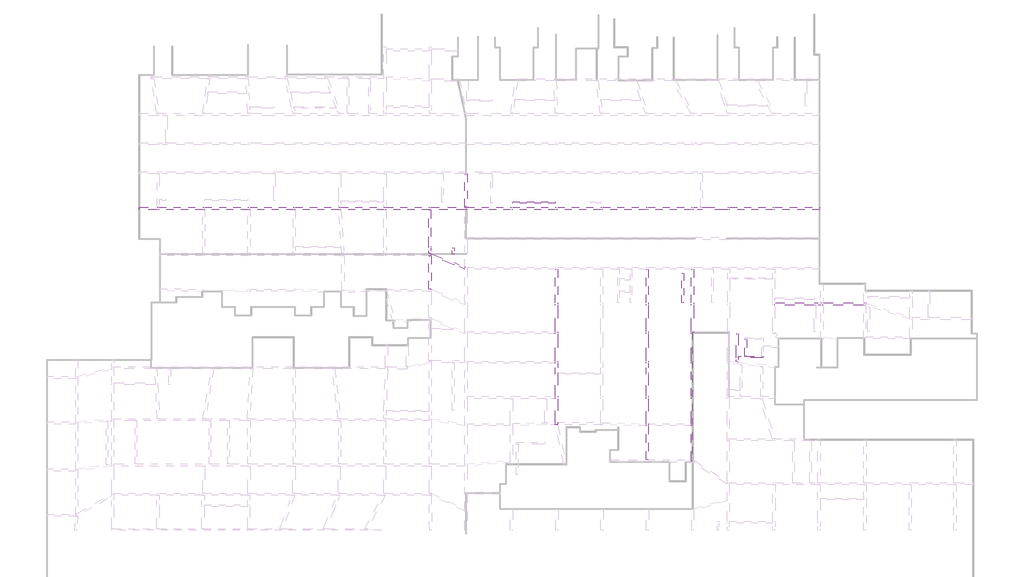
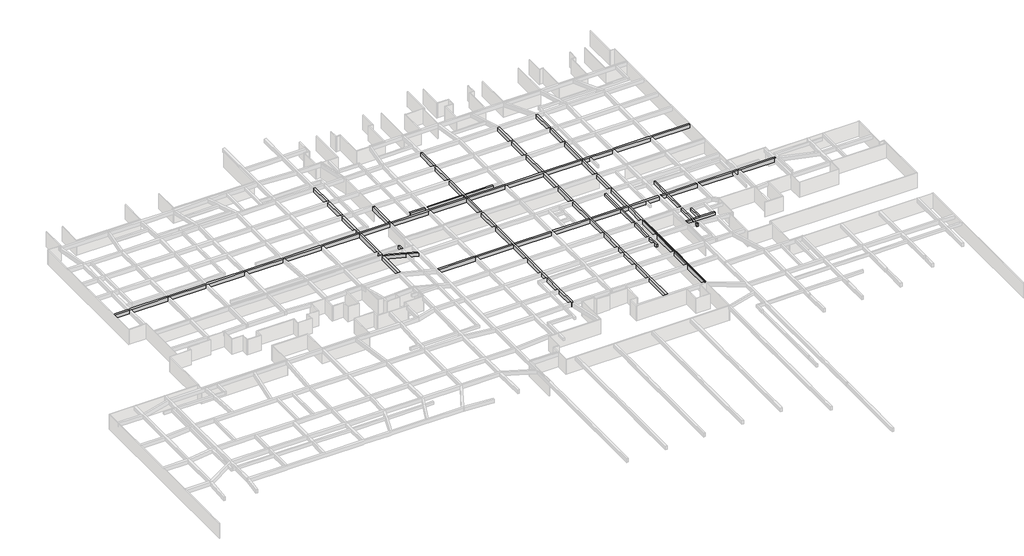
# One storey, part 14 of 16: 15 beams.
"""IFC4 building model written with IfcOpenShell, lengths in millimetres."""

from ifc_helpers import new_model, si_unit, frame, origin, place, context, project, spatial, polyline, outline, extrude, faceted_brep, element, save

model = new_model("IFC4")

# Units and contexts
model_context = context("Model", 3, world=origin())
ifc_project = project(units=[si_unit("LENGTHUNIT", "METRE", prefix="MILLI")], contexts=[model_context])

# Site, building, storey
site = spatial("IfcSite", under=ifc_project)
building = spatial("IfcBuilding", under=site)
storey = spatial("IfcBuildingStorey", under=building, Name="户型图", Elevation=0.0)

# Beams
placement = place(None, origin())
element("IfcBeam", 1, ObjectType="混凝土 - 矩形梁 : KL_beam", at=placement, inside=storey, context=model_context, shape_type="Brep", body=[
    faceted_brep([(204626.2466536, 173512.5884701, 3300.0), (204626.2466536, 173112.5884701, 3300.0), (204626.2466536, 173112.5884701, 2500.0), (204626.2466536, 173512.5884701, 2500.0), (83129.2466536, 173512.5884701, 3300.0), (83129.2466536, 173512.5884701, 2500.0), (83129.2466536, 173112.5884701, 2500.0), (83129.2466536, 173112.5884701, 3300.0), (196626.5590225, 173512.5884701, 3300.0), (196226.5590225, 173512.5884701, 3300.0), (188616.2109037, 173512.5884701, 3300.0), (188216.2109037, 173512.5884701, 3300.0), (183653.5662503, 173512.5884701, 3300.0), (183353.5662503, 173512.5884701, 3300.0), (182116.2109037, 173512.5884701, 3300.0), (181716.2109037, 173512.5884701, 3300.0), (174016.2109037, 173512.5884701, 3300.0), (173616.2109037, 173512.5884701, 3300.0), (165916.2109037, 173512.5884701, 3300.0), (165516.2109037, 173512.5884701, 3300.0), (157816.2109037, 173512.5884701, 3300.0), (157416.2109037, 173512.5884701, 3300.0), (149816.2109037, 173512.5884701, 3300.0), (149416.2109037, 173512.5884701, 3300.0), (141660.1899051, 173512.5884701, 3300.0), (141260.1899051, 173512.5884701, 3300.0), (135216.2109037, 173512.5884701, 3300.0), (134816.2109037, 173512.5884701, 3300.0), (127216.2109037, 173512.5884701, 3300.0), (126816.2109037, 173512.5884701, 3300.0), (119116.2109037, 173512.5884701, 3300.0), (118716.2109037, 173512.5884701, 3300.0), (111016.2109037, 173512.5884701, 3300.0), (110616.2109037, 173512.5884701, 3300.0), (102916.2109037, 173512.5884701, 3300.0), (102516.2109037, 173512.5884701, 3300.0), (94816.2109037, 173512.5884701, 3300.0), (94416.2109037, 173512.5884701, 3300.0), (86694.1615746, 173512.5884701, 3300.0), (86294.1615746, 173512.5884701, 3300.0), (86294.1615746, 173112.5884701, 3300.0), (86694.1615746, 173112.5884701, 3300.0), (94416.2109037, 173112.5884701, 3300.0), (94816.2109037, 173112.5884701, 3300.0), (102516.2109037, 173112.5884701, 3300.0), (102916.2109037, 173112.5884701, 3300.0), (110616.2109037, 173112.5884701, 3300.0), (111016.2109037, 173112.5884701, 3300.0), (118729.7078864, 173112.5884701, 3300.0), (119130.6846457, 173112.5884701, 3300.0), (126816.2109037, 173112.5884701, 3300.0), (127216.2109037, 173112.5884701, 3300.0), (134816.2109037, 173112.5884701, 3300.0), (135216.2109037, 173112.5884701, 3300.0), (141266.2091209, 173112.5884701, 3300.0), (141666.2091209, 173112.5884701, 3300.0), (149416.2109037, 173112.5884701, 3300.0), (149816.2109037, 173112.5884701, 3300.0), (157416.2109037, 173112.5884701, 3300.0), (157816.2109037, 173112.5884701, 3300.0), (165516.2109037, 173112.5884701, 3300.0), (165916.2109037, 173112.5884701, 3300.0), (173616.2109037, 173112.5884701, 3300.0), (174016.2109037, 173112.5884701, 3300.0), (181716.2109037, 173112.5884701, 3300.0), (182116.2109037, 173112.5884701, 3300.0), (183353.5662503, 173112.5884701, 3300.0), (183653.5662503, 173112.5884701, 3300.0), (188216.2109037, 173112.5884701, 3300.0), (188616.2109037, 173112.5884701, 3300.0), (196226.5590225, 173112.5884701, 3300.0), (196626.5590225, 173112.5884701, 3300.0), (86294.1615746, 173112.5884701, 2500.0), (86694.1615746, 173112.5884701, 2500.0), (94416.2109037, 173112.5884701, 2500.0), (94816.2109037, 173112.5884701, 2500.0), (102516.2109037, 173112.5884701, 2500.0), (102916.2109037, 173112.5884701, 2500.0), (110616.2109037, 173112.5884701, 2500.0), (111016.2109037, 173112.5884701, 2500.0), (118729.7078864, 173112.5884701, 2500.0), (119130.6846457, 173112.5884701, 2500.0), (126816.2109037, 173112.5884701, 2500.0), (127216.2109037, 173112.5884701, 2500.0), (134816.2109037, 173112.5884701, 2500.0), (135216.2109037, 173112.5884701, 2500.0), (141266.2091209, 173112.5884701, 2500.0), (141666.2091209, 173112.5884701, 2500.0), (149416.2109037, 173112.5884701, 2500.0), (149816.2109037, 173112.5884701, 2500.0), (157416.2109037, 173112.5884701, 2500.0), (157816.2109037, 173112.5884701, 2500.0), (165516.2109037, 173112.5884701, 2500.0), (165916.2109037, 173112.5884701, 2500.0), (173616.2109037, 173112.5884701, 2500.0), (174016.2109037, 173112.5884701, 2500.0), (181716.2109037, 173112.5884701, 2500.0), (182116.2109037, 173112.5884701, 2500.0), (188216.2109037, 173112.5884701, 2500.0), (188616.2109037, 173112.5884701, 2500.0), (196226.5590225, 173112.5884701, 2500.0), (196626.5590225, 173112.5884701, 2500.0), (86294.1615746, 173512.5884701, 2500.0), (86694.1615746, 173512.5884701, 2500.0), (94416.2109037, 173512.5884701, 2500.0), (94816.2109037, 173512.5884701, 2500.0), (102516.2109037, 173512.5884701, 2500.0), (102916.2109037, 173512.5884701, 2500.0), (110616.2109037, 173512.5884701, 2500.0), (111016.2109037, 173512.5884701, 2500.0), (118716.2109037, 173512.5884701, 2500.0), (119116.2109037, 173512.5884701, 2500.0), (126816.2109037, 173512.5884701, 2500.0), (127216.2109037, 173512.5884701, 2500.0), (134816.2109037, 173512.5884701, 2500.0), (135216.2109037, 173512.5884701, 2500.0), (141260.1899051, 173512.5884701, 2500.0), (141660.1899051, 173512.5884701, 2500.0), (149416.2109037, 173512.5884701, 2500.0), (149816.2109037, 173512.5884701, 2500.0), (157416.2109037, 173512.5884701, 2500.0), (157816.2109037, 173512.5884701, 2500.0), (165516.2109037, 173512.5884701, 2500.0), (165916.2109037, 173512.5884701, 2500.0), (173616.2109037, 173512.5884701, 2500.0), (174016.2109037, 173512.5884701, 2500.0), (181716.2109037, 173512.5884701, 2500.0), (182116.2109037, 173512.5884701, 2500.0), (188216.2109037, 173512.5884701, 2500.0), (188616.2109037, 173512.5884701, 2500.0), (196226.5590225, 173512.5884701, 2500.0), (196626.5590225, 173512.5884701, 2500.0)], [[[0, 1, 2, 3]], [[4, 5, 6, 7]], [[1, 0, 8, 9, 10, 11, 12, 13, 14, 15, 16, 17, 18, 19, 20, 21, 22, 23, 24, 25, 26, 27, 28, 29, 30, 31, 32, 33, 34, 35, 36, 37, 38, 39, 4, 7, 40, 41, 42, 43, 44, 45, 46, 47, 48, 49, 50, 51, 52, 53, 54, 55, 56, 57, 58, 59, 60, 61, 62, 63, 64, 65, 66, 67, 68, 69, 70, 71]], [[2, 1, 71, 70, 69, 68, 67, 66, 65, 64, 63, 62, 61, 60, 59, 58, 57, 56, 55, 54, 53, 52, 51, 50, 49, 48, 47, 46, 45, 44, 43, 42, 41, 40, 7, 6, 72, 73, 74, 75, 76, 77, 78, 79, 80, 81, 82, 83, 84, 85, 86, 87, 88, 89, 90, 91, 92, 93, 94, 95, 96, 97, 98, 99, 100, 101]], [[3, 2, 101, 100, 99, 98, 97, 96, 95, 94, 93, 92, 91, 90, 89, 88, 87, 86, 85, 84, 83, 82, 81, 80, 79, 78, 77, 76, 75, 74, 73, 72, 6, 5, 102, 103, 104, 105, 106, 107, 108, 109, 110, 111, 112, 113, 114, 115, 116, 117, 118, 119, 120, 121, 122, 123, 124, 125, 126, 127, 128, 129, 130, 131]], [[0, 3, 131, 130, 129, 128, 127, 126, 125, 124, 123, 122, 121, 120, 119, 118, 117, 116, 115, 114, 113, 112, 111, 110, 109, 108, 107, 106, 105, 104, 103, 102, 5, 4, 39, 38, 37, 36, 35, 34, 33, 32, 31, 30, 29, 28, 27, 26, 25, 24, 23, 22, 21, 20, 19, 18, 17, 16, 15, 14, 13, 12, 11, 10, 9, 8]]]),
])
element("IfcBeam", 2, ObjectType="混凝土 - 矩形梁 : KL_beam", at=placement, inside=storey, context=model_context, shape_type="Brep", body=[
    faceted_brep([(135228.9386535, 164912.5884701, 3300.0), (134991.8708445, 164912.5884701, 3300.0), (135228.9386535, 164821.5866644, 3300.0), (139049.0511844, 163355.182854, 3300.0), (139349.0511844, 163240.0236434, 3300.0), (141266.2091209, 162504.0956621, 3300.0), (141266.2091209, 162932.5536596, 3300.0), (139349.0511844, 163668.4816409, 3300.0), (139049.0511844, 163783.6408514, 3300.0), (135228.9386535, 165250.0446618, 3300.0), (134991.8708445, 164912.5884701, 2500.0), (135228.9386535, 164821.5866644, 2500.0), (141266.2091209, 162504.0956621, 2500.0), (135228.9386535, 164912.5884701, 2500.0), (135228.9386535, 165250.0446618, 2500.0), (141266.2091209, 162932.5536596, 2500.0)], [[[0, 1, 2, 3, 4, 5, 6, 7, 8, 9]], [[1, 10, 11, 12, 5, 4, 3, 2]], [[10, 13, 14, 15, 12, 11]], [[14, 9, 8, 7, 6, 15]], [[1, 0, 13, 10]], [[13, 0, 9, 14]], [[6, 5, 12, 15]]]),
])
element("IfcBeam", 3, ObjectType="混凝土 - 矩形梁 : KL_beam", at=placement, inside=storey, context=model_context, shape_type="Brep", body=[
    faceted_brep([(135216.2109037, 189895.7397162, 3300.0), (134816.2109037, 189895.7397162, 3300.0), (134816.2109037, 185072.5884701, 3300.0), (135216.2109037, 185072.5884701, 3300.0), (134816.2109037, 189895.7397162, 2500.0), (134816.2109037, 185072.5884701, 2500.0), (135216.2109037, 189895.7397162, 2500.0), (135216.2109037, 185072.5884701, 2500.0)], [[[0, 1, 2, 3]], [[1, 4, 5, 2]], [[4, 6, 7, 5]], [[6, 0, 3, 7]], [[1, 0, 6, 4]], [[3, 2, 5, 7]]]),
    faceted_brep([(135066.0064625, 165312.5884701, 2500.0), (135066.0064625, 165312.5884701, 3300.0), (134828.9386535, 165312.5884701, 3300.0), (134816.2109037, 165312.5884701, 3300.0), (134816.2109037, 165312.5884701, 2500.0), (134828.9386535, 165312.5884701, 2500.0), (135216.2109037, 165254.9303872, 2500.0), (135216.2109037, 165254.9303872, 3300.0), (134816.2109037, 173112.5884701, 3300.0), (135216.2109037, 173112.5884701, 3300.0), (135216.2109037, 173112.5884701, 2500.0), (134816.2109037, 173112.5884701, 2500.0), (135216.2109037, 166295.0298489, 3300.0), (135216.2109037, 166595.0298489, 3300.0), (134816.2109037, 166595.0298489, 3300.0), (134816.2109037, 166295.0298489, 3300.0)], [[[0, 1, 2, 3, 4, 5]], [[1, 0, 6, 7]], [[8, 9, 10, 11]], [[1, 7, 12, 13, 9, 8, 14, 15, 3, 2]], [[4, 3, 15, 14, 8, 11]], [[6, 0, 5, 4, 11, 10]], [[7, 6, 10, 9, 13, 12]]]),
    faceted_brep([(134816.2109037, 184672.5884701, 3300.0), (135216.2109037, 184672.5884701, 3300.0), (135216.2109037, 184672.5884701, 2500.0), (134816.2109037, 184672.5884701, 2500.0), (135216.2109037, 179912.5884701, 3300.0), (134816.2109037, 179912.5884701, 3300.0), (134816.2109037, 179912.5884701, 2500.0), (135216.2109037, 179912.5884701, 2500.0)], [[[0, 1, 2, 3]], [[4, 5, 6, 7]], [[1, 0, 5, 4]], [[0, 3, 6, 5]], [[3, 2, 7, 6]], [[2, 1, 4, 7]]]),
    faceted_brep([(135216.2109037, 179512.5884701, 3300.0), (134816.2109037, 179512.5884701, 3300.0), (134816.2109037, 174724.6482986, 3300.0), (134816.2109037, 174424.6482986, 3300.0), (134816.2109037, 173512.5884701, 3300.0), (135216.2109037, 173512.5884701, 3300.0), (135216.2109037, 174424.6482986, 3300.0), (135216.2109037, 174724.6482986, 3300.0), (134816.2109037, 179512.5884701, 2500.0), (134816.2109037, 173512.5884701, 2500.0), (135216.2109037, 179512.5884701, 2500.0), (135216.2109037, 173512.5884701, 2500.0)], [[[0, 1, 2, 3, 4, 5, 6, 7]], [[1, 8, 9, 4, 3, 2]], [[8, 10, 11, 9]], [[10, 0, 7, 6, 5, 11]], [[1, 0, 10, 8]], [[5, 4, 9, 11]]]),
])
element("IfcBeam", 4, ObjectType="混凝土 - 矩形梁 : KL_beam", at=placement, inside=storey, context=model_context, shape_type="SweptSolid", body=[
    extrude(outline(polyline([(134828.9386535, 164912.5884701), (134991.8708445, 164912.5884701), (135228.9386535, 164821.5866644), (135228.9386535, 158915.0633975), (134828.9386535, 158915.0633975), (134828.9386535, 164912.5884701)])), frame((0.0, 0.0, 2500.0), z_axis=(0.0, 0.0, 1.0), x_axis=(1.0, 0.0, 0.0)), (0.0, 0.0, 1.0), 800.0),
])
element("IfcBeam", 5, ObjectType="混凝土 - 矩形梁 : KL_beam", at=placement, inside=storey, context=model_context, shape_type="Brep", body=[
    faceted_brep([(157816.2109037, 189895.7397162, 3300.0), (157416.2109037, 189895.7397162, 3300.0), (157416.2109037, 185072.5884701, 3300.0), (157816.2109037, 185072.5884701, 3300.0), (157416.2109037, 189895.7397162, 2500.0), (157416.2109037, 185072.5884701, 2500.0), (157816.2109037, 189895.7397162, 2500.0), (157816.2109037, 185072.5884701, 2500.0)], [[[0, 1, 2, 3]], [[1, 4, 5, 2]], [[4, 6, 7, 5]], [[6, 0, 3, 7]], [[1, 0, 6, 4]], [[3, 2, 5, 7]]]),
    faceted_brep([(157416.2109037, 184672.5884701, 3300.0), (157816.2109037, 184672.5884701, 3300.0), (157816.2109037, 184672.5884701, 2500.0), (157416.2109037, 184672.5884701, 2500.0), (157816.2109037, 179912.5884701, 3300.0), (157416.2109037, 179912.5884701, 3300.0), (157416.2109037, 179912.5884701, 2500.0), (157816.2109037, 179912.5884701, 2500.0)], [[[0, 1, 2, 3]], [[4, 5, 6, 7]], [[1, 0, 5, 4]], [[0, 3, 6, 5]], [[3, 2, 7, 6]], [[2, 1, 4, 7]]]),
    faceted_brep([(157816.2109037, 173512.5884701, 3300.0), (157816.2109037, 174220.6993439, 3300.0), (157816.2109037, 174520.6993439, 3300.0), (157816.2109037, 179512.5884701, 3300.0), (157416.2109037, 179512.5884701, 3300.0), (157416.2109037, 174520.6993439, 3300.0), (157416.2109037, 174220.6993439, 3300.0), (157416.2109037, 173512.5884701, 3300.0), (157416.2109037, 179512.5884701, 2500.0), (157416.2109037, 173512.5884701, 2500.0), (157816.2109037, 179512.5884701, 2500.0), (157816.2109037, 173512.5884701, 2500.0)], [[[0, 1, 2, 3, 4, 5, 6, 7]], [[7, 6, 5, 4, 8, 9]], [[9, 8, 10, 11]], [[3, 2, 1, 0, 11, 10]], [[4, 3, 10, 8]], [[0, 7, 9, 11]]]),
    faceted_brep([(157416.2109037, 173112.5884701, 3300.0), (157816.2109037, 173112.5884701, 3300.0), (157816.2109037, 173112.5884701, 2500.0), (157416.2109037, 173112.5884701, 2500.0), (157816.2109037, 168162.578939, 3300.0), (157416.2109037, 168162.578939, 3300.0), (157416.2109037, 168162.578939, 2500.0), (157816.2109037, 168162.578939, 2500.0)], [[[0, 1, 2, 3]], [[4, 5, 6, 7]], [[1, 0, 5, 4]], [[0, 3, 6, 5]], [[3, 2, 7, 6]], [[2, 1, 4, 7]]]),
    faceted_brep([(157416.2109037, 162447.0169772, 3300.0), (157816.2109037, 162447.0169772, 3300.0), (157816.2109037, 162447.0169772, 2500.0), (157416.2109037, 162447.0169772, 2500.0), (157816.2109037, 134700.2382994, 3300.0), (157618.4857796, 134695.7397162, 3300.0), (157455.0445029, 134692.0211489, 3300.0), (157416.2109037, 134691.1376184, 3300.0), (157416.2109037, 134691.1376184, 2500.0), (157455.0445029, 134692.0211489, 2500.0), (157618.4857796, 134695.7397162, 2500.0), (157816.2109037, 134700.2382994, 2500.0), (157816.2109037, 135095.7397162, 3300.0), (157816.2109037, 139362.5884701, 3300.0), (157816.2109037, 139762.5884701, 3300.0), (157816.2109037, 143695.3207545, 3300.0), (157816.2109037, 143995.3207545, 3300.0), (157816.2109037, 145662.5884701, 3300.0), (157816.2109037, 146062.5884701, 3300.0), (157816.2109037, 150902.424794, 3300.0), (157816.2109037, 151302.424794, 3300.0), (157816.2109037, 156044.0267812, 3300.0), (157816.2109037, 156444.0267812, 3300.0), (157416.2109037, 156444.0267812, 3300.0), (157416.2109037, 156044.0267812, 3300.0), (157416.2109037, 151302.424794, 3300.0), (157416.2109037, 150902.424794, 3300.0), (157416.2109037, 146062.5884701, 3300.0), (157416.2109037, 145662.5884701, 3300.0), (157416.2109037, 143995.3207545, 3300.0), (157416.2109037, 143695.3207545, 3300.0), (157416.2109037, 139762.5884701, 3300.0), (157416.2109037, 139362.5884701, 3300.0), (157416.2109037, 135091.241133, 3300.0), (157416.2109037, 156444.0267812, 2500.0), (157416.2109037, 156044.0267812, 2500.0), (157416.2109037, 151302.424794, 2500.0), (157416.2109037, 150902.424794, 2500.0), (157416.2109037, 146062.5884701, 2500.0), (157416.2109037, 145662.5884701, 2500.0), (157416.2109037, 139762.5884701, 2500.0), (157416.2109037, 139362.5884701, 2500.0), (157416.2109037, 135091.241133, 2500.0), (157816.2109037, 156444.0267812, 2500.0), (157816.2109037, 156044.0267812, 2500.0), (157816.2109037, 151302.424794, 2500.0), (157816.2109037, 150902.424794, 2500.0), (157816.2109037, 146062.5884701, 2500.0), (157816.2109037, 145662.5884701, 2500.0), (157816.2109037, 139762.5884701, 2500.0), (157816.2109037, 139362.5884701, 2500.0), (157816.2109037, 135095.7397162, 2500.0)], [[[0, 1, 2, 3]], [[4, 5, 6, 7, 8, 9, 10, 11]], [[7, 6, 5, 4, 12, 13, 14, 15, 16, 17, 18, 19, 20, 21, 22, 1, 0, 23, 24, 25, 26, 27, 28, 29, 30, 31, 32, 33]], [[8, 7, 33, 32, 31, 30, 29, 28, 27, 26, 25, 24, 23, 0, 3, 34, 35, 36, 37, 38, 39, 40, 41, 42]], [[11, 10, 9, 8, 42, 41, 40, 39, 38, 37, 36, 35, 34, 3, 2, 43, 44, 45, 46, 47, 48, 49, 50, 51]], [[4, 11, 51, 50, 49, 48, 47, 46, 45, 44, 43, 2, 1, 22, 21, 20, 19, 18, 17, 16, 15, 14, 13, 12]]]),
    faceted_brep([(157816.2109037, 162847.0169772, 3300.0), (157416.2109037, 162847.0169772, 3300.0), (157416.2109037, 162847.0169772, 2500.0), (157816.2109037, 162847.0169772, 2500.0), (157416.2109037, 167762.578939, 3300.0), (157816.2109037, 167762.578939, 3300.0), (157816.2109037, 167762.578939, 2500.0), (157416.2109037, 167762.578939, 2500.0)], [[[0, 1, 2, 3]], [[4, 5, 6, 7]], [[1, 0, 5, 4]], [[2, 1, 4, 7]], [[3, 2, 7, 6]], [[0, 3, 6, 5]]]),
])
element("IfcBeam", 6, ObjectType="混凝土 - 矩形梁 : KL_beam", at=placement, inside=storey, context=model_context, shape_type="Brep", body=[
    faceted_brep([(174016.2109037, 189895.7397162, 3300.0), (173616.2109037, 189895.7397162, 3300.0), (173616.2109037, 185072.5884701, 3300.0), (174016.2109037, 185072.5884701, 3300.0), (173616.2109037, 189895.7397162, 2500.0), (173616.2109037, 185072.5884701, 2500.0), (174016.2109037, 189895.7397162, 2500.0), (174016.2109037, 185072.5884701, 2500.0)], [[[0, 1, 2, 3]], [[1, 4, 5, 2]], [[4, 6, 7, 5]], [[6, 0, 3, 7]], [[1, 0, 6, 4]], [[3, 2, 5, 7]]]),
    faceted_brep([(173616.2109037, 184672.5884701, 3300.0), (174016.2109037, 184672.5884701, 3300.0), (174016.2109037, 184672.5884701, 2500.0), (173616.2109037, 184672.5884701, 2500.0), (174016.2109037, 179912.5884701, 3300.0), (173616.2109037, 179912.5884701, 3300.0), (173616.2109037, 179912.5884701, 2500.0), (174016.2109037, 179912.5884701, 2500.0)], [[[0, 1, 2, 3]], [[4, 5, 6, 7]], [[1, 0, 5, 4]], [[0, 3, 6, 5]], [[3, 2, 7, 6]], [[2, 1, 4, 7]]]),
    faceted_brep([(174016.2109037, 179512.5884701, 3300.0), (173616.2109037, 179512.5884701, 3300.0), (173616.2109037, 173512.5884701, 3300.0), (174016.2109037, 173512.5884701, 3300.0), (173616.2109037, 179512.5884701, 2500.0), (173616.2109037, 173512.5884701, 2500.0), (174016.2109037, 179512.5884701, 2500.0), (174016.2109037, 173512.5884701, 2500.0)], [[[0, 1, 2, 3]], [[1, 4, 5, 2]], [[4, 6, 7, 5]], [[6, 0, 3, 7]], [[1, 0, 6, 4]], [[3, 2, 5, 7]]]),
    faceted_brep([(173616.2109037, 173112.5884701, 3300.0), (174016.2109037, 173112.5884701, 3300.0), (174016.2109037, 173112.5884701, 2500.0), (173616.2109037, 173112.5884701, 2500.0), (174016.2109037, 168162.578939, 3300.0), (173616.2109037, 168162.578939, 3300.0), (173616.2109037, 168162.578939, 2500.0), (174016.2109037, 168162.578939, 2500.0)], [[[0, 1, 2, 3]], [[4, 5, 6, 7]], [[1, 0, 5, 4]], [[0, 3, 6, 5]], [[3, 2, 7, 6]], [[2, 1, 4, 7]]]),
    faceted_brep([(173616.2109037, 162447.0169772, 3300.0), (174016.2109037, 162447.0169772, 3300.0), (174016.2109037, 162447.0169772, 2500.0), (173616.2109037, 162447.0169772, 2500.0), (173616.2109037, 156444.0267812, 3300.0), (173616.2109037, 156044.0267812, 3300.0), (173616.2109037, 151302.424794, 3300.0), (173616.2109037, 150902.424794, 3300.0), (173616.2109037, 146062.5884701, 3300.0), (173616.2109037, 145662.5884701, 3300.0), (173616.2109037, 143995.3207545, 3300.0), (173616.2109037, 143695.3207545, 3300.0), (173616.2109037, 139762.5884701, 3300.0), (173616.2109037, 139362.5884701, 3300.0), (173616.2109037, 134875.3714487, 3300.0), (173616.2109037, 134475.2157459, 3300.0), (173616.2109037, 128412.5884701, 3300.0), (174016.2109037, 128412.5884701, 3300.0), (174016.2109037, 134469.7126829, 3300.0), (174016.2109037, 134869.7126829, 3300.0), (174016.2109037, 139362.5884701, 3300.0), (174016.2109037, 139762.5884701, 3300.0), (174016.2109037, 143695.3207545, 3300.0), (174016.2109037, 143995.3207545, 3300.0), (174016.2109037, 145662.5884701, 3300.0), (174016.2109037, 146062.5884701, 3300.0), (174016.2109037, 150902.424794, 3300.0), (174016.2109037, 151302.424794, 3300.0), (174016.2109037, 156044.0267812, 3300.0), (174016.2109037, 156444.0267812, 3300.0), (173616.2109037, 156444.0267812, 2500.0), (173616.2109037, 156044.0267812, 2500.0), (173616.2109037, 151302.424794, 2500.0), (173616.2109037, 150902.424794, 2500.0), (173616.2109037, 146062.5884701, 2500.0), (173616.2109037, 145662.5884701, 2500.0), (173616.2109037, 139762.5884701, 2500.0), (173616.2109037, 139362.5884701, 2500.0), (173616.2109037, 134875.3714487, 2500.0), (173616.2109037, 134475.2157459, 2500.0), (173616.2109037, 128412.5884701, 2500.0), (174016.2109037, 156444.0267812, 2500.0), (174016.2109037, 156044.0267812, 2500.0), (174016.2109037, 151302.424794, 2500.0), (174016.2109037, 150902.424794, 2500.0), (174016.2109037, 146062.5884701, 2500.0), (174016.2109037, 145662.5884701, 2500.0), (174016.2109037, 139762.5884701, 2500.0), (174016.2109037, 139362.5884701, 2500.0), (174016.2109037, 134869.7126829, 2500.0), (174016.2109037, 134469.7126829, 2500.0), (174016.2109037, 128412.5884701, 2500.0)], [[[0, 1, 2, 3]], [[1, 0, 4, 5, 6, 7, 8, 9, 10, 11, 12, 13, 14, 15, 16, 17, 18, 19, 20, 21, 22, 23, 24, 25, 26, 27, 28, 29]], [[0, 3, 30, 31, 32, 33, 34, 35, 36, 37, 38, 39, 40, 16, 15, 14, 13, 12, 11, 10, 9, 8, 7, 6, 5, 4]], [[3, 2, 41, 42, 43, 44, 45, 46, 47, 48, 49, 50, 51, 40, 39, 38, 37, 36, 35, 34, 33, 32, 31, 30]], [[2, 1, 29, 28, 27, 26, 25, 24, 23, 22, 21, 20, 19, 18, 17, 51, 50, 49, 48, 47, 46, 45, 44, 43, 42, 41]], [[17, 16, 40, 51]]]),
    faceted_brep([(174016.2109037, 162847.0169772, 3300.0), (173616.2109037, 162847.0169772, 3300.0), (173616.2109037, 162847.0169772, 2500.0), (174016.2109037, 162847.0169772, 2500.0), (173616.2109037, 167762.578939, 3300.0), (174016.2109037, 167762.578939, 3300.0), (174016.2109037, 167762.578939, 2500.0), (173616.2109037, 167762.578939, 2500.0)], [[[0, 1, 2, 3]], [[4, 5, 6, 7]], [[1, 0, 5, 4]], [[2, 1, 4, 7]], [[3, 2, 7, 6]], [[0, 3, 6, 5]]]),
])
element("IfcBeam", 7, ObjectType="混凝土 - 矩形梁 : KL_beam", at=placement, inside=storey, context=model_context, shape_type="Brep", body=[
    faceted_brep([(182116.2109037, 128212.6640931, 2500.0), (182116.2109037, 128212.6640931, 3300.0), (182017.7367524, 128212.6640931, 3300.0), (182017.7367524, 128212.6640931, 2500.0), (182116.2109037, 128323.4502804, 3300.0), (182116.2109037, 134469.7126829, 3300.0), (182116.2109037, 134869.7126829, 3300.0), (182116.2109037, 139362.5884701, 3300.0), (182116.2109037, 139762.5884701, 3300.0), (182116.2109037, 145662.5884701, 3300.0), (182116.2109037, 146062.5884701, 3300.0), (182116.2109037, 150902.424794, 3300.0), (182116.2109037, 151052.5884701, 3300.0), (182017.7367524, 151052.5884701, 3300.0), (182116.2109037, 128323.4502804, 2500.0), (182116.2109037, 134469.7126829, 2500.0), (182116.2109037, 134869.7126829, 2500.0), (182116.2109037, 139362.5884701, 2500.0), (182116.2109037, 139762.5884701, 2500.0), (182116.2109037, 145662.5884701, 2500.0), (182116.2109037, 146062.5884701, 2500.0), (182116.2109037, 150902.424794, 2500.0), (182116.2109037, 151052.5884701, 2500.0), (182017.7367524, 151052.5884701, 2500.0)], [[[0, 1, 2, 3]], [[2, 1, 4, 5, 6, 7, 8, 9, 10, 11, 12, 13]], [[1, 0, 14, 15, 16, 17, 18, 19, 20, 21, 22, 12, 11, 10, 9, 8, 7, 6, 5, 4]], [[3, 2, 13, 23]], [[13, 12, 22, 23]], [[0, 3, 23, 22, 21, 20, 19, 18, 17, 16, 15, 14]]]),
    faceted_brep([(181716.2109037, 128212.6640931, 2500.0), (181716.2109037, 128212.6640931, 3300.0), (181716.2109037, 128412.5884701, 3300.0), (181716.2109037, 134469.7126829, 3300.0), (181716.2109037, 134869.7126829, 3300.0), (181716.2109037, 139362.5884701, 3300.0), (181716.2109037, 139762.5884701, 3300.0), (181716.2109037, 145662.5884701, 3300.0), (181716.2109037, 146062.5884701, 3300.0), (181716.2109037, 150902.424794, 3300.0), (181716.2109037, 151302.424794, 3300.0), (181716.2109037, 156044.0267812, 3300.0), (181716.2109037, 156444.0267812, 3300.0), (181716.2109037, 162447.0169772, 3300.0), (181716.2109037, 162447.0169772, 2500.0), (181716.2109037, 156444.0267812, 2500.0), (181716.2109037, 156044.0267812, 2500.0), (181716.2109037, 151302.424794, 2500.0), (181716.2109037, 150902.424794, 2500.0), (181716.2109037, 146062.5884701, 2500.0), (181716.2109037, 145662.5884701, 2500.0), (181716.2109037, 139762.5884701, 2500.0), (181716.2109037, 139362.5884701, 2500.0), (181716.2109037, 134869.7126829, 2500.0), (181716.2109037, 134469.7126829, 2500.0), (181716.2109037, 128412.5884701, 2500.0), (182116.2109037, 162447.0169772, 2500.0), (182116.2109037, 156444.0267812, 2500.0), (182116.2109037, 156044.0267812, 2500.0), (182116.2109037, 151302.424794, 2500.0), (182116.2109037, 151172.5884701, 2500.0), (181897.7367524, 151172.5884701, 2500.0), (181897.7367524, 128212.6640931, 2500.0), (182116.2109037, 162447.0169772, 3300.0), (181897.7367524, 128212.6640931, 3300.0), (181897.7367524, 151172.5884701, 3300.0), (182116.2109037, 151172.5884701, 3300.0), (182017.7367524, 151172.5884701, 3300.0), (182116.2109037, 151302.424794, 3300.0), (182116.2109037, 156044.0267812, 3300.0), (182116.2109037, 156444.0267812, 3300.0)], [[[0, 1, 2, 3, 4, 5, 6, 7, 8, 9, 10, 11, 12, 13, 14, 15, 16, 17, 18, 19, 20, 21, 22, 23, 24, 25]], [[0, 25, 24, 23, 22, 21, 20, 19, 18, 17, 16, 15, 14, 26, 27, 28, 29, 30, 31, 32]], [[13, 33, 26, 14]], [[34, 32, 31, 35]], [[1, 0, 32, 34]], [[35, 31, 30, 36, 37]], [[13, 12, 11, 10, 9, 8, 7, 6, 5, 4, 3, 2, 1, 34, 35, 37, 36, 38, 39, 40, 33]], [[26, 33, 40, 39, 38, 36, 30, 29, 28, 27]]]),
    faceted_brep([(181716.2109037, 189895.7397162, 3300.0), (182116.2109037, 189895.7397162, 3300.0), (182116.2109037, 189895.7397162, 2500.0), (181716.2109037, 189895.7397162, 2500.0), (182116.2109037, 185072.5884701, 3300.0), (181716.2109037, 185072.5884701, 3300.0), (181716.2109037, 185072.5884701, 2500.0), (182116.2109037, 185072.5884701, 2500.0)], [[[0, 1, 2, 3]], [[4, 5, 6, 7]], [[1, 0, 5, 4]], [[0, 3, 6, 5]], [[3, 2, 7, 6]], [[2, 1, 4, 7]]]),
    faceted_brep([(181716.2109037, 184672.5884701, 3300.0), (182116.2109037, 184672.5884701, 3300.0), (182116.2109037, 184672.5884701, 2500.0), (181716.2109037, 184672.5884701, 2500.0), (182116.2109037, 179912.5884701, 3300.0), (181716.2109037, 179912.5884701, 3300.0), (181716.2109037, 179912.5884701, 2500.0), (182116.2109037, 179912.5884701, 2500.0)], [[[0, 1, 2, 3]], [[4, 5, 6, 7]], [[1, 0, 5, 4]], [[0, 3, 6, 5]], [[3, 2, 7, 6]], [[2, 1, 4, 7]]]),
    faceted_brep([(181716.2109037, 179512.5884701, 3300.0), (182116.2109037, 179512.5884701, 3300.0), (182116.2109037, 179512.5884701, 2500.0), (181716.2109037, 179512.5884701, 2500.0), (182116.2109037, 173512.5884701, 3300.0), (181716.2109037, 173512.5884701, 3300.0), (181716.2109037, 173512.5884701, 2500.0), (182116.2109037, 173512.5884701, 2500.0)], [[[0, 1, 2, 3]], [[4, 5, 6, 7]], [[1, 0, 5, 4]], [[0, 3, 6, 5]], [[3, 2, 7, 6]], [[2, 1, 4, 7]]]),
    faceted_brep([(181716.2109037, 173112.5884701, 3300.0), (182116.2109037, 173112.5884701, 3300.0), (182116.2109037, 173112.5884701, 2500.0), (181716.2109037, 173112.5884701, 2500.0), (182116.2109037, 168162.578939, 3300.0), (181716.2109037, 168162.578939, 3300.0), (181716.2109037, 168162.578939, 2500.0), (182116.2109037, 168162.578939, 2500.0)], [[[0, 1, 2, 3]], [[4, 5, 6, 7]], [[1, 0, 5, 4]], [[0, 3, 6, 5]], [[3, 2, 7, 6]], [[2, 1, 4, 7]]]),
    faceted_brep([(182116.2109037, 162847.0169772, 3300.0), (181716.2109037, 162847.0169772, 3300.0), (181716.2109037, 162847.0169772, 2500.0), (182116.2109037, 162847.0169772, 2500.0), (181716.2109037, 167762.578939, 3300.0), (182116.2109037, 167762.578939, 3300.0), (182116.2109037, 167762.578939, 2500.0), (181716.2109037, 167762.578939, 2500.0)], [[[0, 1, 2, 3]], [[4, 5, 6, 7]], [[1, 0, 5, 4]], [[2, 1, 4, 7]], [[3, 2, 7, 6]], [[0, 3, 6, 5]]]),
])
element("IfcBeam", 8, ObjectType="混凝土 - 矩形梁 : KL_beam", at=placement, inside=storey, context=model_context, shape_type="Brep", body=[
    faceted_brep([(141666.2091209, 156444.0267812, 3300.0), (141666.2091209, 156044.0267812, 3300.0), (149416.2109037, 156044.0267812, 3300.0), (149816.2109037, 156044.0267812, 3300.0), (157416.2109037, 156044.0267812, 3300.0), (157416.2109037, 156444.0267812, 3300.0), (149816.2109037, 156444.0267812, 3300.0), (149416.2109037, 156444.0267812, 3300.0), (141666.2091209, 156044.0267812, 2500.0), (149416.2109037, 156044.0267812, 2500.0), (149816.2109037, 156044.0267812, 2500.0), (157416.2109037, 156044.0267812, 2500.0), (141666.2091209, 156444.0267812, 2500.0), (149416.2109037, 156444.0267812, 2500.0), (149816.2109037, 156444.0267812, 2500.0), (157416.2109037, 156444.0267812, 2500.0)], [[[0, 1, 2, 3, 4, 5, 6, 7]], [[1, 8, 9, 10, 11, 4, 3, 2]], [[8, 12, 13, 14, 15, 11, 10, 9]], [[12, 0, 7, 6, 5, 15, 14, 13]], [[1, 0, 12, 8]], [[5, 4, 11, 15]]]),
    faceted_brep([(157816.2109037, 156044.0267812, 3300.0), (157816.2109037, 156444.0267812, 3300.0), (157816.2109037, 156444.0267812, 2500.0), (157816.2109037, 156044.0267812, 2500.0), (165516.2109037, 156444.0267812, 3300.0), (165516.2109037, 156044.0267812, 3300.0), (165516.2109037, 156044.0267812, 2500.0), (165516.2109037, 156444.0267812, 2500.0)], [[[0, 1, 2, 3]], [[4, 5, 6, 7]], [[1, 0, 5, 4]], [[0, 3, 6, 5]], [[3, 2, 7, 6]], [[2, 1, 4, 7]]]),
    faceted_brep([(165916.2109037, 156444.0267812, 3300.0), (165916.2109037, 156044.0267812, 3300.0), (173616.2109037, 156044.0267812, 3300.0), (173616.2109037, 156444.0267812, 3300.0), (171091.2109037, 156444.0267812, 3300.0), (170791.2109037, 156444.0267812, 3300.0), (168841.2109037, 156444.0267812, 3300.0), (168541.2109037, 156444.0267812, 3300.0), (165916.2109037, 156044.0267812, 2500.0), (173616.2109037, 156044.0267812, 2500.0), (165916.2109037, 156444.0267812, 2500.0), (173616.2109037, 156444.0267812, 2500.0)], [[[0, 1, 2, 3, 4, 5, 6, 7]], [[1, 8, 9, 2]], [[8, 10, 11, 9]], [[10, 0, 7, 6, 5, 4, 3, 11]], [[1, 0, 10, 8]], [[3, 2, 9, 11]]]),
    faceted_brep([(174016.2109037, 156044.0267812, 3300.0), (174016.2109037, 156444.0267812, 3300.0), (174016.2109037, 156444.0267812, 2500.0), (174016.2109037, 156044.0267812, 2500.0), (181716.2109037, 156444.0267812, 3300.0), (181716.2109037, 156044.0267812, 3300.0), (181716.2109037, 156044.0267812, 2500.0), (181716.2109037, 156444.0267812, 2500.0), (180041.8640388, 156044.0267812, 3300.0), (180341.8640388, 156044.0267812, 3300.0), (180341.8640388, 156444.0267812, 3300.0), (180041.8640388, 156444.0267812, 3300.0)], [[[0, 1, 2, 3]], [[4, 5, 6, 7]], [[1, 0, 8, 9, 5, 4, 10, 11]], [[0, 3, 6, 5, 9, 8]], [[3, 2, 7, 6]], [[2, 1, 11, 10, 4, 7]]]),
    faceted_brep([(182116.2109037, 156044.0267812, 3300.0), (182116.2109037, 156444.0267812, 3300.0), (182116.2109037, 156444.0267812, 2500.0), (182116.2109037, 156044.0267812, 2500.0), (188216.2109037, 156444.0267812, 3300.0), (188216.2109037, 156044.0267812, 3300.0), (188216.2109037, 156044.0267812, 2500.0), (188216.2109037, 156444.0267812, 2500.0), (185353.3391382, 156044.0267812, 3300.0), (185653.3391382, 156044.0267812, 3300.0), (185653.3391382, 156444.0267812, 3300.0), (185353.3391382, 156444.0267812, 3300.0)], [[[0, 1, 2, 3]], [[4, 5, 6, 7]], [[1, 0, 8, 9, 5, 4, 10, 11]], [[0, 3, 6, 5, 9, 8]], [[3, 2, 7, 6]], [[2, 1, 11, 10, 4, 7]]]),
    faceted_brep([(188616.2109037, 156044.0267812, 3300.0), (188616.2109037, 156444.0267812, 3300.0), (188616.2109037, 156444.0267812, 2500.0), (188616.2109037, 156044.0267812, 2500.0), (196226.5590225, 156444.0267812, 3300.0), (196226.5590225, 156044.0267812, 3300.0), (196226.5590225, 156044.0267812, 2500.0), (196226.5590225, 156444.0267812, 2500.0), (189774.1000448, 156044.0267812, 3300.0), (190074.1000448, 156044.0267812, 3300.0), (190074.1000448, 156444.0267812, 3300.0), (189774.1000448, 156444.0267812, 3300.0)], [[[0, 1, 2, 3]], [[4, 5, 6, 7]], [[1, 0, 8, 9, 5, 4, 10, 11]], [[0, 3, 6, 5, 9, 8]], [[3, 2, 7, 6]], [[2, 1, 11, 10, 4, 7]]]),
    faceted_brep([(196626.5590225, 156044.0267812, 3300.0), (196626.5590225, 156444.0267812, 3300.0), (196626.5590225, 156444.0267812, 2500.0), (196626.5590225, 156044.0267812, 2500.0), (212866.2091209, 156444.0267812, 3300.0), (212866.2091209, 156392.0189962, 3300.0), (212866.2091209, 156044.0267812, 3300.0), (212866.2091209, 156044.0267812, 2500.0), (212866.2091209, 156392.0189962, 2500.0), (212866.2091209, 156444.0267812, 2500.0), (212466.2091209, 156444.0267812, 3300.0), (205246.2265287, 156444.0267812, 3300.0), (204846.2265287, 156444.0267812, 3300.0), (203953.3391382, 156444.0267812, 3300.0), (203653.3391382, 156444.0267812, 3300.0), (203653.3391382, 156044.0267812, 3300.0), (203953.3391382, 156044.0267812, 3300.0), (204846.2265287, 156044.0267812, 3300.0), (205246.2265287, 156044.0267812, 3300.0), (212466.2091209, 156044.0267812, 3300.0), (204846.2265287, 156044.0267812, 2500.0), (205246.2265287, 156044.0267812, 2500.0), (212466.2091209, 156044.0267812, 2500.0), (204846.2265287, 156444.0267812, 2500.0), (205246.2265287, 156444.0267812, 2500.0), (212466.2091209, 156444.0267812, 2500.0)], [[[0, 1, 2, 3]], [[4, 5, 6, 7, 8, 9]], [[6, 5, 4, 10, 11, 12, 13, 14, 1, 0, 15, 16, 17, 18, 19]], [[7, 6, 19, 18, 17, 16, 15, 0, 3, 20, 21, 22]], [[9, 8, 7, 22, 21, 20, 3, 2, 23, 24, 25]], [[4, 9, 25, 24, 23, 2, 1, 14, 13, 12, 11, 10]]]),
])
element("IfcBeam", 9, ObjectType="混凝土 - 矩形梁 : KL_beam", at=placement, inside=storey, context=model_context, shape_type="SweptSolid", body=[
    extrude(outline(polyline([(141260.1899051, 179512.5884701), (141660.1899051, 179512.5884701), (141660.1899051, 173512.5884701), (141260.1899051, 173512.5884701), (141260.1899051, 179512.5884701)])), frame((0.0, 0.0, 2500.0), z_axis=(0.0, 0.0, 1.0), x_axis=(1.0, 0.0, 0.0)), (0.0, 0.0, 1.0), 800.0),
])
element("IfcBeam", 10, ObjectType="混凝土 - 矩形梁 : L_beam", at=placement, inside=storey, context=model_context, shape_type="SweptSolid", body=[
    extrude(outline(polyline([(163696.1090193, 174220.6993439), (157816.2109037, 174220.6993439), (157816.2109037, 174520.6993439), (163696.1090193, 174520.6993439), (163696.1090193, 174220.6993439)])), frame((0.0, 0.0, 2700.0), z_axis=(0.0, 0.0, 1.0), x_axis=(1.0, 0.0, 0.0)), (0.0, 0.0, 1.0), 600.0),
    extrude(outline(polyline([(146146.1090193, 174220.6993439), (146146.1090193, 174520.6993439), (149416.2109037, 174520.6993439), (149416.2109037, 174220.6993439), (146146.1090193, 174220.6993439)])), frame((0.0, 0.0, 2700.0), z_axis=(0.0, 0.0, 1.0), x_axis=(1.0, 0.0, 0.0)), (0.0, 0.0, 1.0), 600.0),
    extrude(outline(polyline([(157416.2109037, 174520.6993439), (157416.2109037, 174220.6993439), (149816.2109037, 174220.6993439), (149816.2109037, 174520.6993439), (157416.2109037, 174520.6993439)])), frame((0.0, 0.0, 2700.0), z_axis=(0.0, 0.0, 1.0), x_axis=(1.0, 0.0, 0.0)), (0.0, 0.0, 1.0), 600.0),
])
element("IfcBeam", 11, ObjectType="混凝土 - 矩形梁 : L_beam", at=placement, inside=storey, context=model_context, shape_type="Brep", body=[
    faceted_brep([(190074.1000448, 145082.5631037, 3300.0), (189774.1000448, 145082.5631037, 3300.0), (189774.1000448, 145082.5631037, 2700.0), (190074.1000448, 145082.5631037, 2700.0), (190074.1000448, 145481.1706052, 3300.0), (189774.1000448, 145511.9520424, 3300.0), (189774.1000448, 145511.9520424, 2700.0), (190074.1000448, 145481.1706052, 2700.0)], [[[0, 1, 2, 3]], [[1, 0, 4, 5]], [[2, 1, 5, 6]], [[3, 2, 6, 7]], [[0, 3, 7, 4]], [[5, 4, 7, 6]]]),
    faceted_brep([(189774.1000448, 160683.8998965, 3300.0), (190074.1000448, 160683.8998965, 3300.0), (190074.1000448, 160683.8998965, 2700.0), (189774.1000448, 160683.8998965, 2700.0), (190074.1000448, 156444.0267812, 3300.0), (189774.1000448, 156444.0267812, 3300.0), (189774.1000448, 156444.0267812, 2700.0), (190074.1000448, 156444.0267812, 2700.0), (190074.1000448, 157037.5884701, 3300.0), (190074.1000448, 157337.5884701, 3300.0), (190074.1000448, 157337.5884701, 2700.0), (190074.1000448, 157037.5884701, 2700.0)], [[[0, 1, 2, 3]], [[4, 5, 6, 7]], [[1, 0, 5, 4, 8, 9]], [[0, 3, 6, 5]], [[3, 2, 10, 11, 7, 6]], [[2, 1, 9, 8, 4, 7, 11, 10]]]),
    faceted_brep([(189774.1000448, 156044.0267812, 3300.0), (190074.1000448, 156044.0267812, 3300.0), (190074.1000448, 156044.0267812, 2700.0), (189774.1000448, 156044.0267812, 2700.0), (190074.1000448, 151302.424794, 3300.0), (189774.1000448, 151302.424794, 3300.0), (189774.1000448, 151302.424794, 2700.0), (190074.1000448, 151302.424794, 2700.0)], [[[0, 1, 2, 3]], [[4, 5, 6, 7]], [[1, 0, 5, 4]], [[0, 3, 6, 5]], [[3, 2, 7, 6]], [[2, 1, 4, 7]]]),
    faceted_brep([(189774.1000448, 150902.424794, 3300.0), (190074.1000448, 150902.424794, 3300.0), (190074.1000448, 150902.424794, 2700.0), (189774.1000448, 150902.424794, 2700.0), (190074.1000448, 145883.2706412, 3300.0), (189774.1000448, 145914.0520783, 3300.0), (189774.1000448, 145914.0520783, 2700.0), (190074.1000448, 145883.2706412, 2700.0), (189774.1000448, 146955.8638084, 3300.0), (189774.1000448, 146655.8638084, 3300.0), (190074.1000448, 146655.8638084, 3300.0), (190074.1000448, 146955.8638084, 3300.0), (189774.1000448, 146955.8638084, 2700.0), (189774.1000448, 146655.8638084, 2700.0), (190074.1000448, 146955.8638084, 2700.0), (190074.1000448, 146655.8638084, 2700.0)], [[[0, 1, 2, 3]], [[4, 5, 6, 7]], [[1, 0, 8, 9, 5, 4, 10, 11]], [[0, 3, 12, 13, 6, 5, 9, 8]], [[3, 2, 14, 15, 7, 6, 13, 12]], [[2, 1, 11, 10, 4, 7, 15, 14]]]),
])
element("IfcBeam", 12, ObjectType="混凝土 - 矩形梁 : L_beam", at=placement, inside=storey, context=model_context, shape_type="Brep", body=[
    faceted_brep([(180341.8640388, 143046.1128776, 3300.0), (180041.8640388, 143046.1128776, 3300.0), (180041.8640388, 143046.1128776, 2700.0), (180341.8640388, 143046.1128776, 2700.0), (180341.8640388, 145662.5884701, 3300.0), (180041.8640388, 145662.5884701, 3300.0), (180041.8640388, 143995.3207545, 3300.0), (180041.8640388, 143695.3207545, 3300.0), (180041.8640388, 145662.5884701, 2700.0), (180041.8640388, 143995.3207545, 2700.0), (180041.8640388, 143695.3207545, 2700.0), (180341.8640388, 145662.5884701, 2700.0)], [[[0, 1, 2, 3]], [[1, 0, 4, 5, 6, 7]], [[2, 1, 7, 6, 5, 8, 9, 10]], [[3, 2, 10, 9, 8, 11]], [[0, 3, 11, 4]], [[5, 4, 11, 8]]]),
    faceted_brep([(180341.8640388, 161771.1128776, 3300.0), (180341.8640388, 161771.1128776, 2700.0), (180041.8640388, 161771.1128776, 2700.0), (180041.8640388, 161771.1128776, 3300.0), (180341.8640388, 156444.0267812, 3300.0), (180041.8640388, 156444.0267812, 3300.0), (180041.8640388, 156444.0267812, 2700.0), (180341.8640388, 156444.0267812, 2700.0)], [[[0, 1, 2, 3]], [[4, 5, 6, 7]], [[0, 3, 5, 4]], [[3, 2, 6, 5]], [[2, 1, 7, 6]], [[1, 0, 4, 7]]]),
    faceted_brep([(180041.8640388, 156044.0267812, 3300.0), (180341.8640388, 156044.0267812, 3300.0), (180341.8640388, 156044.0267812, 2700.0), (180041.8640388, 156044.0267812, 2700.0), (180341.8640388, 151302.424794, 3300.0), (180041.8640388, 151302.424794, 3300.0), (180041.8640388, 151302.424794, 2700.0), (180341.8640388, 151302.424794, 2700.0)], [[[0, 1, 2, 3]], [[4, 5, 6, 7]], [[1, 0, 5, 4]], [[0, 3, 6, 5]], [[3, 2, 7, 6]], [[2, 1, 4, 7]]]),
    faceted_brep([(180041.8640388, 150902.424794, 3300.0), (180341.8640388, 150902.424794, 3300.0), (180341.8640388, 150902.424794, 2700.0), (180041.8640388, 150902.424794, 2700.0), (180341.8640388, 146062.5884701, 3300.0), (180041.8640388, 146062.5884701, 3300.0), (180041.8640388, 146062.5884701, 2700.0), (180341.8640388, 146062.5884701, 2700.0)], [[[0, 1, 2, 3]], [[4, 5, 6, 7]], [[1, 0, 5, 4]], [[0, 3, 6, 5]], [[3, 2, 7, 6]], [[2, 1, 4, 7]]]),
])
element("IfcBeam", 13, ObjectType="混凝土 - 矩形梁 : L_beam", at=placement, inside=storey, context=model_context, shape_type="SweptSolid", body=[
    extrude(outline(polyline([(139349.0511844, 165162.578939), (139049.0511844, 165162.578939), (139049.0511844, 166295.0298489), (139349.0511844, 166295.0298489), (139349.0511844, 165162.578939)])), frame((0.0, 0.0, 2700.0), z_axis=(0.0, 0.0, 1.0), x_axis=(1.0, 0.0, 0.0)), (0.0, 0.0, 1.0), 600.0),
])
element("IfcBeam", 14, ObjectType="混凝土 - 矩形梁 : L_beam", at=placement, inside=storey, context=model_context, shape_type="Brep", body=[
    faceted_brep([(188516.2109037, 146955.8638084, 3300.0), (188516.2109037, 146655.8638084, 3300.0), (189774.1000448, 146655.8638084, 3300.0), (189774.1000448, 146955.8638084, 3300.0), (188516.2109037, 146655.8638084, 2700.0), (189774.1000448, 146655.8638084, 2700.0), (188516.2109037, 146955.8638084, 2700.0), (189774.1000448, 146955.8638084, 2700.0)], [[[0, 1, 2, 3]], [[1, 4, 5, 2]], [[4, 6, 7, 5]], [[6, 0, 3, 7]], [[1, 0, 6, 4]], [[3, 2, 5, 7]]]),
    faceted_brep([(190074.1000448, 146655.8638084, 3300.0), (190074.1000448, 146955.8638084, 3300.0), (190074.1000448, 146955.8638084, 2700.0), (190074.1000448, 146655.8638084, 2700.0), (194566.2109037, 146655.8638084, 3300.0), (194566.2109037, 146955.8638084, 3300.0), (194266.2109037, 146955.8638084, 3300.0), (191566.2109037, 146955.8638084, 3300.0), (191266.2109037, 146955.8638084, 3300.0), (194566.2109037, 146655.8638084, 2700.0), (194566.2109037, 146955.8638084, 2700.0), (191266.2109037, 146955.8638084, 2700.0), (191566.2109037, 146955.8638084, 2700.0), (194266.2109037, 146955.8638084, 2700.0)], [[[0, 1, 2, 3]], [[4, 5, 6, 7, 8, 1, 0]], [[9, 4, 0, 3]], [[10, 9, 3, 2, 11, 12, 13]], [[5, 10, 13, 12, 11, 2, 1, 8, 7, 6]], [[5, 4, 9, 10]]]),
])
element("IfcBeam", 15, ObjectType="混凝土 - 矩形梁 : L_beam", at=placement, inside=storey, context=model_context, shape_type="SweptSolid", body=[
    extrude(outline(polyline([(191266.2109037, 149955.8638084), (191566.2109037, 149955.8638084), (191566.2109037, 146955.8638084), (191266.2109037, 146955.8638084), (191266.2109037, 149955.8638084)])), frame((0.0, 0.0, 2700.0), z_axis=(0.0, 0.0, 1.0), x_axis=(1.0, 0.0, 0.0)), (0.0, 0.0, 1.0), 600.0),
])

save(model, "model.ifc")

# Revit data of these elements
# Type "混凝土 - 矩形梁 : KL_beam"
#   Length [instance default] = 1524 mm
#   b = 400 mm
#   h = 800 mm
#   Structural Material [instance default] = 混凝土 - 现场浇注混凝土
#   Assembly Code = ""
# Type "混凝土 - 矩形梁 : L_beam"
#   Length [instance default] = 1524 mm
#   b = 300 mm
#   h = 600 mm
#   Structural Material [instance default] = none
#   Assembly Code = ""
# Elements 1, 2, 3, 4, 5, 6, 7, 8, 9 (IfcBeam, "混凝土 - 矩形梁 : KL_beam")
#   Comments = ""
#   Structural Material = none
#   Phase Created = 新构造
# Elements 10, 11, 12, 13, 14, 15 (IfcBeam, "混凝土 - 矩形梁 : L_beam")
#   Comments = ""
#   Structural Material = none
#   Phase Created = 新构造
# Materials
#   "混凝土 - 现场浇注混凝土": class "混凝土", colour RGB 192 192 192, transparency 0
